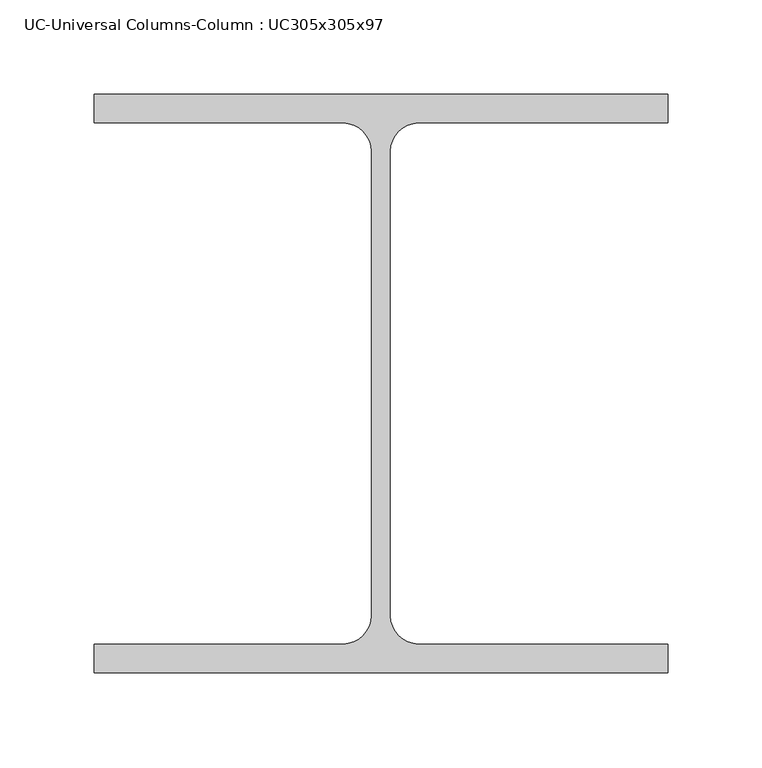
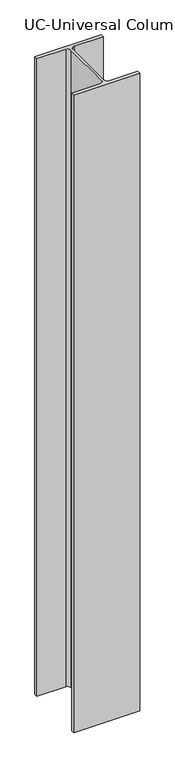
"""IFC4 building model written with IfcOpenShell, lengths in millimetres: column geometry, UC-Universal Columns-Column : UC305x305x97."""

from ifc_helpers import new_model, si_unit, point, frame, frame_2d, origin, place, context, project, spatial, polyline, circle_curve, trimmed, segment, composite_curve, outline, extrude, source, transform, mapped, element, save


def uc_universal_columns_column_uc305x305x97_d51453b7(model_context):
    return source(origin(), model_context, "Body", "SweptSolid", [
        extrude(outline(composite_curve([segment(polyline([(152.65, 153.95), (152.65, 138.55), (20.15, 138.55)]), True, "CONTINUOUS"), segment(trimmed(circle_curve(frame_2d((20.15, 123.35)), 15.2), [point((20.15, 138.55))], [point((4.95, 123.35))], True, "CARTESIAN"), True, "CONTINUOUS"), segment(polyline([(4.95, 123.35), (4.95, -123.35)]), True, "CONTINUOUS"), segment(trimmed(circle_curve(frame_2d((20.15, -123.35)), 15.2), [point((4.95, -123.35))], [point((20.15, -138.55))], True, "CARTESIAN"), True, "CONTINUOUS"), segment(polyline([(20.15, -138.55), (152.65, -138.55), (152.65, -153.95), (-152.65, -153.95), (-152.65, -138.55), (-20.15, -138.55)]), True, "CONTINUOUS"), segment(trimmed(circle_curve(frame_2d((-20.15, -123.35)), 15.2), [point((-20.15, -138.55))], [point((-4.95, -123.35))], True, "CARTESIAN"), True, "CONTINUOUS"), segment(polyline([(-4.95, -123.35), (-4.95, 123.35)]), True, "CONTINUOUS"), segment(trimmed(circle_curve(frame_2d((-20.15, 123.35)), 15.2), [point((-4.95, 123.35))], [point((-20.15, 138.55))], True, "CARTESIAN"), True, "CONTINUOUS"), segment(polyline([(-20.15, 138.55), (-152.65, 138.55), (-152.65, 153.95), (152.65, 153.95)]), True, "CONTINUOUS")], self_intersect=False)), frame((0.0, 0.0, 2900.0), z_axis=(0.0, 0.0, 1.0), x_axis=(1.0, 0.0, 0.0)), (0.0, 0.0, 1.0), 3105.0),
    ])


if __name__ == "__main__":
    model = new_model("IFC4")
    model_context = context("Model", 3, world=origin())
    ifc_project = project(units=[si_unit("LENGTHUNIT", "METRE", prefix="MILLI")], contexts=[model_context])
    site = spatial("IfcSite", under=ifc_project)
    building = spatial("IfcBuilding", under=site)
    placement = place(None, origin())
    uc_universal_columns_column_uc305x305x97_shape = uc_universal_columns_column_uc305x305x97_d51453b7(model_context)
    element("IfcColumn", 1, ObjectType="UC-Universal Columns-Column : UC305x305x97", at=placement, inside=building, context=model_context, shape_type="MappedRepresentation", body=[
        mapped(uc_universal_columns_column_uc305x305x97_shape, transform((0.0, 0.0, 0.0), x_axis=(1.0, 0.0, 0.0), y_axis=(0.0, 1.0, 0.0), z_axis=(0.0, 0.0, 1.0))),
    ])
    save(model, "model.ifc")

# Revit data of these elements
# Type "UC-Universal Columns-Column : UC305x305x97"
#   Section Name Key = "UC305x305x97"
#   Cost = 2
#   Width = 30.53 cm
#   Web Thickness = 0.99 cm
#   Web Fillet = 1.52 cm
#   Warping Constant = 1560000.0 cm⁶
#   Torsional Moment of Inertia = 91.20 cm⁴
#   Section Area = 123.0 cm²
#   Plastic Modulus weak axis = 726.0 cm³
#   Plastic Modulus strong axis = 1592.0 cm³
#   Nominal Weight = 96.8996 kgf/m
#   Moment of Inertia weak axis = 7308.00 cm⁴
#   Moment of Inertia strong axis = 22249.00 cm⁴
#   Height = 30.79 cm
#   Flange Thickness = 1.54 cm
#   Elastic Modulus weak axis = 479.0 cm³
#   Elastic Modulus strong axis = 1445.0 cm³
#   Centroid Vertical = 15.395 cm
#   Centroid Horizontal = 15.265 cm
#   Bolt Spacing = 14.0 cm
#   Structural Material [instance default] = Metal - Steel 43-275
#   Type Comments = ""
#   Assembly Code = ""
# Element 1 (IfcColumn, "UC-Universal Columns-Column : UC305x305x97")
#   Materials on its faces: "Metal - Steel 43-275"
# Materials
#   "Metal - Steel 43-275": class "Metal", colour RGB 247 247 247, transparency 0, Cost = 0
